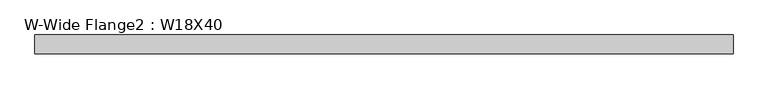
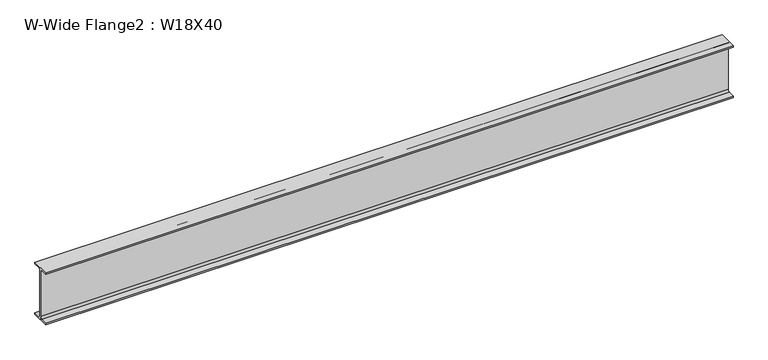
"""IFC4 building model written with IfcOpenShell, lengths in millimetres: beam geometry, W-Wide Flange2 : W18X40."""

from ifc_helpers import new_model, si_unit, point, frame, frame_2d, origin, place, context, project, spatial, polyline, circle_curve, trimmed, segment, composite_curve, outline, extrude, source, transform, mapped, element, save


def w_wide_flange2_w18x40_de17c711(model_context):
    return source(origin(), model_context, "Body", "SweptSolid", [
        extrude(outline(composite_curve([segment(polyline([(76.454, -213.995), (76.454, -227.33), (-76.454, -227.33), (-76.454, -213.995), (-20.828, -213.995)]), True, "CONTINUOUS"), segment(trimmed(circle_curve(frame_2d((-20.828, -197.1675)), 16.8275), [point((-20.828, -213.995))], [point((-4.0005, -197.1675))], True, "CARTESIAN"), True, "CONTINUOUS"), segment(polyline([(-4.0005, -197.1675), (-4.0005, 197.1675)]), True, "CONTINUOUS"), segment(trimmed(circle_curve(frame_2d((-20.828, 197.1675)), 16.8275), [point((-4.0005, 197.1675))], [point((-20.828, 213.995))], True, "CARTESIAN"), True, "CONTINUOUS"), segment(polyline([(-20.828, 213.995), (-76.454, 213.995), (-76.454, 227.33), (76.454, 227.33), (76.454, 213.995), (20.828, 213.995)]), True, "CONTINUOUS"), segment(trimmed(circle_curve(frame_2d((20.828, 197.1675)), 16.8275), [point((20.828, 213.995))], [point((4.0005, 197.1675))], True, "CARTESIAN"), True, "CONTINUOUS"), segment(polyline([(4.0005, 197.1675), (4.0005, -197.1675)]), True, "CONTINUOUS"), segment(trimmed(circle_curve(frame_2d((20.828, -197.1675)), 16.8275), [point((4.0005, -197.1675))], [point((20.828, -213.995))], True, "CARTESIAN"), True, "CONTINUOUS"), segment(polyline([(20.828, -213.995), (76.454, -213.995)]), True, "CONTINUOUS")], self_intersect=False)), frame((-2805.1125, 0.0, 0.0), z_axis=(1.0, 0.0, 0.0), x_axis=(0.0, 1.0, 0.0)), (0.0, 0.0, 1.0), 5667.375),
    ])


if __name__ == "__main__":
    model = new_model("IFC4")
    model_context = context("Model", 3, world=origin())
    ifc_project = project(units=[si_unit("LENGTHUNIT", "METRE", prefix="MILLI")], contexts=[model_context])
    site = spatial("IfcSite", under=ifc_project)
    building = spatial("IfcBuilding", under=site)
    placement = place(None, origin())
    w_wide_flange2_w18x40_shape = w_wide_flange2_w18x40_de17c711(model_context)
    element("IfcBeam", 1, ObjectType="W-Wide Flange2 : W18X40", at=placement, inside=building, context=model_context, shape_type="MappedRepresentation", body=[
        mapped(w_wide_flange2_w18x40_shape, transform((0.0, 0.0, 0.0), x_axis=(1.0, 0.0, 0.0), y_axis=(0.0, 1.0, 0.0), z_axis=(0.0, 0.0, 1.0))),
    ])
    save(model, "model.ifc")

# Revit data of these elements
# Type "W-Wide Flange2 : W18X40"
#   Assembly Code = "B10"
#   W = 40
#   Length [instance default] = 5' - 0"
#   bf = 0' - 6.02"
#   d = 1' - 5.9"
#   k = 0' - 1 3/16"
#   k2 = 0' - 0.6625"
#   tf = 0' - 0.525"
#   tw = 0' - 0.315"
#   A = 0.0819444 SF
#   Structural Material [instance default] = Steel ASTM A992
# Element 1 (IfcBeam, "W-Wide Flange2 : W18X40")
#   Materials on its faces: "Steel ASTM A992"
# Materials
#   "Steel ASTM A992": class "Metal", colour RGB 199 199 199, transparency 0, Description = "Structural steel 50ksi", Cost = 0
